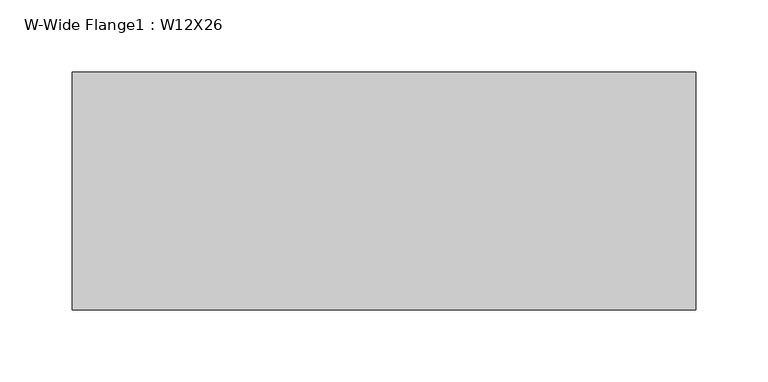
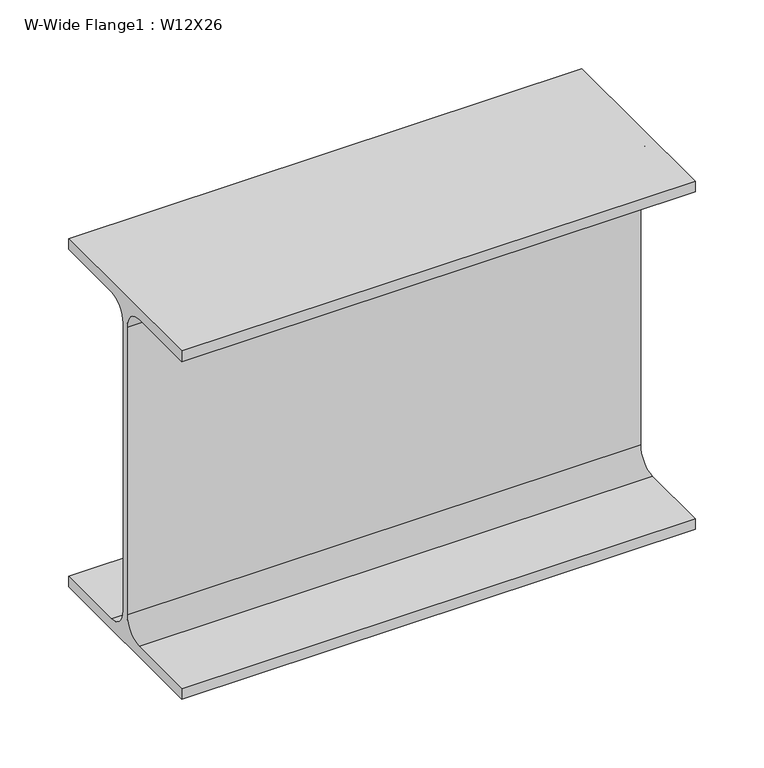
"""IFC4 building model written with IfcOpenShell, lengths in millimetres: beam geometry, W-Wide Flange1 : W12X26."""

from ifc_helpers import new_model, si_unit, point, frame, frame_2d, origin, place, context, project, spatial, polyline, circle_curve, trimmed, segment, composite_curve, outline, extrude, source, transform, mapped, element, save


def w_wide_flange1_w12x26_c28b8588(model_context):
    return source(origin(), model_context, "Body", "SweptSolid", [
        extrude(outline(composite_curve([segment(polyline([(82.423, -145.288), (82.423, -154.94), (-82.423, -154.94), (-82.423, -145.288), (-20.2565, -145.288)]), True, "CONTINUOUS"), segment(trimmed(circle_curve(frame_2d((-20.2565, -127.9525)), 17.3355), [point((-20.2565, -145.288))], [point((-2.921, -127.9525))], True, "CARTESIAN"), True, "CONTINUOUS"), segment(polyline([(-2.921, -127.9525), (-2.921, 127.9525)]), True, "CONTINUOUS"), segment(trimmed(circle_curve(frame_2d((-20.2565, 127.9525)), 17.3355), [point((-2.921, 127.9525))], [point((-20.2565, 145.288))], True, "CARTESIAN"), True, "CONTINUOUS"), segment(polyline([(-20.2565, 145.288), (-82.423, 145.288), (-82.423, 154.94), (82.423, 154.94), (82.423, 145.288), (20.2565, 145.288)]), True, "CONTINUOUS"), segment(trimmed(circle_curve(frame_2d((20.2565, 127.9525)), 17.3355), [point((20.2565, 145.288))], [point((2.921, 127.9525))], True, "CARTESIAN"), True, "CONTINUOUS"), segment(polyline([(2.921, 127.9525), (2.921, -127.9525)]), True, "CONTINUOUS"), segment(trimmed(circle_curve(frame_2d((20.2565, -127.9525)), 17.3355), [point((2.921, -127.9525))], [point((20.2565, -145.288))], True, "CARTESIAN"), True, "CONTINUOUS"), segment(polyline([(20.2565, -145.288), (82.423, -145.288)]), True, "CONTINUOUS")], self_intersect=False)), frame((-100.0165073, 0.0, 0.0), z_axis=(1.0, 0.0, 0.0), x_axis=(0.0, 1.0, 0.0)), (0.0, 0.0, 1.0), 431.8900125),
    ])


if __name__ == "__main__":
    model = new_model("IFC4")
    model_context = context("Model", 3, world=origin())
    ifc_project = project(units=[si_unit("LENGTHUNIT", "METRE", prefix="MILLI")], contexts=[model_context])
    site = spatial("IfcSite", under=ifc_project)
    building = spatial("IfcBuilding", under=site)
    placement = place(None, origin())
    w_wide_flange1_w12x26_shape = w_wide_flange1_w12x26_c28b8588(model_context)
    element("IfcBeam", 1, ObjectType="W-Wide Flange1 : W12X26", at=placement, inside=building, context=model_context, shape_type="MappedRepresentation", body=[
        mapped(w_wide_flange1_w12x26_shape, transform((0.0, 0.0, 0.0), x_axis=(1.0, 0.0, 0.0), y_axis=(0.0, 1.0, 0.0), z_axis=(0.0, 0.0, 1.0))),
    ])
    save(model, "model.ifc")

# Revit data of these elements
# Type "W-Wide Flange1 : W12X26"
#   Assembly Code = "B10"
#   W = 26
#   Start Extension Calculation [instance default] = 10' - 0"
#   Start Extension [instance default] = -0' - 0 1/2"
#   End Extension Calculation [instance default] = 10' - 0"
#   End Extension [instance default] = -0' - 0 1/2"
#   Length [instance default] = 5' - 0"
#   bf = 0' - 6.49"
#   d = 1' - 0.2"
#   k = 0' - 1 1/16"
#   k2 = 0' - 0.6825"
#   tf = 0' - 0.38"
#   tw = 0' - 0.23"
#   A = 0.053125 SF
#   Structural Material [instance default] = Metal - Steel - ASTM A992
# Element 1 (IfcBeam, "W-Wide Flange1 : W12X26")
#   Materials on its faces: "Metal - Steel - ASTM A992"
# Materials
#   "Metal - Steel - ASTM A992": class "Metal", colour RGB 199 199 199, transparency 0
